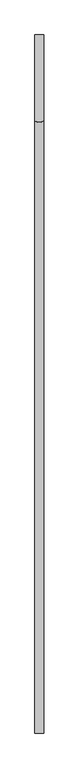
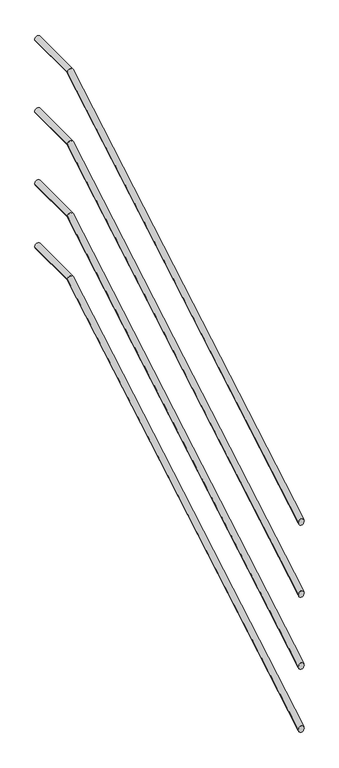
"""IFC4 building model written with IfcOpenShell, lengths in millimetres: railing geometry."""

import ifcopenshell
import ifcopenshell.guid

model = None  # the IFC model being written
_history = None  # IfcOwnerHistory: only IFC2X3 demands one
_inside = {}  # id of a spatial element -> (the spatial element, [elements in it])
_under = {}  # id of a project, library or spatial element -> (it, [spatial elements below it])
_declared = {}  # id of a project -> (the project, [libraries it declares])
_typed = {}  # id of a type object -> (the type object, [elements of that type])
_made_of = {}  # id of a material, layer set ... -> (it, [elements and type objects made of it])


def new_model(schema):
    """Start an empty IFC model of exactly this schema.

    Asked for "IFC4X3", IfcOpenShell would pick the latest addendum, in which some entities
    have other attributes; the version numbers below select the first issue.
    IFC2X3 requires an IfcOwnerHistory on every rooted entity: one is made here for all.
    """
    global model, _history
    if schema == "IFC4X3":
        model = ifcopenshell.file(schema_version=(4, 3, 0, 0))
    else:
        model = ifcopenshell.file(schema=schema)
    _inside.clear()
    _under.clear()
    _declared.clear()
    _typed.clear()
    _made_of.clear()
    _history = None
    if model.schema == "IFC2X3":
        org = make("IfcOrganization", Name="unknown")
        user = make(
            "IfcPersonAndOrganization",
            ThePerson=make("IfcPerson", FamilyName="unknown"),
            TheOrganization=org,
        )
        app = make(
            "IfcApplication",
            ApplicationDeveloper=org,
            Version="unknown",
            ApplicationFullName="unknown",
            ApplicationIdentifier="unknown",
        )
        _history = make(
            "IfcOwnerHistory",
            OwningUser=user,
            OwningApplication=app,
            ChangeAction="ADDED",
            CreationDate=0,
        )
    return model


def make(cls, **values):
    """One entity of the class cls with the attributes given. An attribute that is None is left unset."""
    return model.create_entity(
        cls, **{name: value for name, value in values.items() if value is not None}
    )


def rooted(cls, **values):
    """An entity with a GlobalId (a new one), such as an element, a storey or a relation."""
    return make(cls, GlobalId=ifcopenshell.guid.new(), OwnerHistory=_history, **values)


def si_unit(unit_type, name, prefix=None):
    """IfcSIUnit, for example si_unit("LENGTHUNIT", "METRE", prefix="MILLI")."""
    return make("IfcSIUnit", UnitType=unit_type, Prefix=prefix, Name=name)


def assignment(units):
    """IfcUnitAssignment: the units of a project."""
    return None if units is None else make("IfcUnitAssignment", Units=units)


def point(xyz):
    """IfcCartesianPoint."""
    return None if xyz is None else make("IfcCartesianPoint", Coordinates=xyz)


def direction(xyz):
    """IfcDirection."""
    return None if xyz is None else make("IfcDirection", DirectionRatios=xyz)


def frame(location, z_axis=None, x_axis=None):
    """IfcAxis2Placement3D, a coordinate frame: its origin and axes. An axis left out is left unset."""
    return make(
        "IfcAxis2Placement3D",
        Location=point(location),
        Axis=direction(z_axis),
        RefDirection=direction(x_axis),
    )


def origin():
    """The frame at (0, 0, 0) with its axes left unset."""
    return frame((0.0, 0.0, 0.0))


def place(relative_to, where):
    """IfcLocalPlacement: puts the frame where relative to a parent placement (None: the world)."""
    return make(
        "IfcLocalPlacement", PlacementRelTo=relative_to, RelativePlacement=where
    )


def context(
    kind, dimensions, precision=None, world=None, true_north=None, identifier=None
):
    """IfcGeometricRepresentationContext, for example the 3D "Model" context."""
    return make(
        "IfcGeometricRepresentationContext",
        ContextIdentifier=identifier,
        ContextType=kind,
        CoordinateSpaceDimension=dimensions,
        Precision=precision,
        WorldCoordinateSystem=world,
        TrueNorth=true_north,
    )


def project(units=None, contexts=None):
    """IfcProject with its units and contexts."""
    return rooted(
        "IfcProject",
        Name="project",
        RepresentationContexts=contexts,
        UnitsInContext=assignment(units),
    )


def spatial(cls, under=None, at=None, **own):
    """A site, building, storey or space (cls), placed at a placement, below another one or the project."""
    s = rooted(cls, ObjectPlacement=at, **own)
    if under is not None:
        _under.setdefault(under.id(), (under, []))[1].append(s)
    return s


def circle_curve(where, radius):
    """IfcCircle in the frame where."""
    return make("IfcCircle", Position=where, Radius=radius)


def ellipse_curve(where, semi_axis1, semi_axis2):
    """IfcEllipse in the frame where."""
    return make(
        "IfcEllipse", Position=where, SemiAxis1=semi_axis1, SemiAxis2=semi_axis2
    )


def shape(context_of_items, identifier, shape_type, items):
    """IfcShapeRepresentation: the items that make up one representation, for example the "Body"."""
    return make(
        "IfcShapeRepresentation",
        ContextOfItems=context_of_items,
        RepresentationIdentifier=identifier,
        RepresentationType=shape_type,
        Items=items,
    )


def source(mapping_origin, context_of_items, identifier, shape_type, items):
    """IfcRepresentationMap: a shape defined once, which mapped items show again and again."""
    return make(
        "IfcRepresentationMap",
        MappingOrigin=mapping_origin,
        MappedRepresentation=shape(context_of_items, identifier, shape_type, items),
    )


def transform(
    local_origin,
    x_axis=None,
    y_axis=None,
    z_axis=None,
    scale=None,
    scale2=None,
    scale3=None,
    uniform=True,
):
    """IfcCartesianTransformationOperator3D, or its non-uniform kind. x_axis, y_axis, z_axis: its Axis1, 2, 3."""
    if uniform:
        return make(
            "IfcCartesianTransformationOperator3D",
            Axis1=direction(x_axis),
            Axis2=direction(y_axis),
            LocalOrigin=point(local_origin),
            Scale=scale,
            Axis3=direction(z_axis),
        )
    return make(
        "IfcCartesianTransformationOperator3DnonUniform",
        Axis1=direction(x_axis),
        Axis2=direction(y_axis),
        LocalOrigin=point(local_origin),
        Scale=scale,
        Axis3=direction(z_axis),
        Scale2=scale2,
        Scale3=scale3,
    )


def mapped(mapping_source, mapping_target):
    """IfcMappedItem: shows the shape of a source again, moved by a transform."""
    return make(
        "IfcMappedItem", MappingSource=mapping_source, MappingTarget=mapping_target
    )


def made_of(thing, what):
    """Note that an element or type object is made of a material, layer set ...; save() writes the relation."""
    if what is not None:
        _made_of.setdefault(what.id(), (what, []))[1].append(thing)
    return thing


def element(
    cls,
    number,
    at=None,
    inside=None,
    cuts=None,
    type_object=None,
    material=None,
    context=None,
    identifier="Body",
    shape_type=None,
    held_by="IfcProductDefinitionShape",
    body=None,
    shapes=None,
    **own,
):
    """One element of the class cls, such as IfcWall. Its Tag is "e" and its number.

    at: its placement. inside: the storey or other place that contains it. cuts: it is an
    opening in that element (IfcRelVoidsElement). A single representation is given by context,
    identifier, shape_type and body (its items); several are given by shapes. held_by: the class
    of the entity that holds the representations. save() writes the other relations.
    """
    e = rooted(cls, Tag="e%d" % number, ObjectPlacement=at, **own)
    if body is not None:
        shapes = [shape(context, identifier, shape_type, body)]
    if shapes is not None:
        e.Representation = make(held_by, Representations=shapes)
    if inside is not None:
        _inside.setdefault(inside.id(), (inside, []))[1].append(e)
    if cuts is not None:
        rooted(
            "IfcRelVoidsElement", RelatingBuildingElement=cuts, RelatedOpeningElement=e
        )
    if type_object is not None:
        _typed.setdefault(type_object.id(), (type_object, []))[1].append(e)
    return made_of(e, material)


def aggregate(whole, parts):
    """IfcRelAggregates: a whole, such as a stair, and the parts it consists of."""
    return rooted("IfcRelAggregates", RelatingObject=whole, RelatedObjects=parts)


def save(model, path):
    """Write the relations noted so far, then the file.

    IfcRelAggregates (storeys below a building ...), IfcRelContainedInSpatialStructure (elements
    in a storey), IfcRelDefinesByType, IfcRelAssociatesMaterial and IfcRelDeclares: one each for
    every whole, place, type object, material and project.
    """
    for whole, parts in _under.values():
        aggregate(whole, parts)
    for where, things in _inside.values():
        rooted(
            "IfcRelContainedInSpatialStructure",
            RelatedElements=things,
            RelatingStructure=where,
        )
    for kind, things in _typed.values():
        rooted("IfcRelDefinesByType", RelatedObjects=things, RelatingType=kind)
    for what, things in _made_of.values():
        rooted("IfcRelAssociatesMaterial", RelatedObjects=things, RelatingMaterial=what)
    for by, libraries in _declared.values():
        rooted("IfcRelDeclares", RelatingContext=by, RelatedDefinitions=libraries)
    model.write(path)


def plane_surface(at):
    """IfcPlane: the flat surface through the origin of the frame at, square to its z axis."""
    return make("IfcPlane", Position=at)


def cylinder_surface(at, radius):
    """IfcCylindricalSurface: all points at the distance radius from the z axis of the frame at."""
    return make("IfcCylindricalSurface", Position=at, Radius=radius)


def advanced_brep(points, edges, surfaces, faces):
    """IfcAdvancedBrep: a solid bounded by faces that lie on surfaces and meet in shared edges.

    An edge is (start, end): straight between two places in points (the first is 0);
    or (start, end, curve); or (start, end, curve, False) where it runs against its curve.
    A face is (place in surfaces, loops), or (place, loops, False) where it looks against
    its surface's normal. A loop lists edges by number (the first is 1), with a minus sign
    where the edge is run from its end to its start. The first loop is the outer one.
    """
    corners = [point(p) for p in points]
    vertices = [make("IfcVertexPoint", VertexGeometry=c) for c in corners]
    made = []
    for start, end, *more in edges:
        made.append(
            make(
                "IfcEdgeCurve",
                EdgeStart=vertices[start],
                EdgeEnd=vertices[end],
                EdgeGeometry=more[0] if more else make("IfcPolyline", Points=[corners[start], corners[end]]),
                SameSense=more[1] if len(more) > 1 else True,
            )
        )
    hull = []
    for where, loops, *sense in faces:
        bounds = []
        for j, loop in enumerate(loops):
            ring = [make("IfcOrientedEdge", EdgeElement=made[abs(k) - 1], Orientation=k > 0) for k in loop]
            bounds.append(
                make(
                    "IfcFaceOuterBound" if j == 0 else "IfcFaceBound",
                    Bound=make("IfcEdgeLoop", EdgeList=ring),
                    Orientation=True,
                )
            )
        hull.append(make("IfcAdvancedFace", Bounds=bounds, FaceSurface=surfaces[where], SameSense=sense[0] if sense else True))
    return make("IfcAdvancedBrep", Outer=make("IfcClosedShell", CfsFaces=hull))


def railing_ea222afd(model_context):
    return source(origin(), model_context, "Body", "AdvancedBrep", [
        advanced_brep(
        [(-3259.6, 13399.5208589, 7257.5963084), (-3289.6, 13399.5208589, 7257.5963084), (-3259.6, 15503.576096, 8484.9618634), (-3289.6, 15503.576096, 8484.9618634), (-3259.6, 15799.5208589, 8484.9618634), (-3289.6, 15799.5208589, 8484.9618634)],
        [
            (0, 1, ellipse_curve(frame((-3274.6, 13399.5208589, 7257.5963084), z_axis=(0.0, -1.0, 0.0), x_axis=(0.0, 0.0, -1.0)), 17.365555, 15.0)),
            (1, 0, ellipse_curve(frame((-3274.6, 13399.5208589, 7257.5963084), z_axis=(0.0, -1.0, 0.0), x_axis=(0.0, 0.0, -1.0)), 17.365555, 15.0)),
            (0, 2),
            (2, 3, ellipse_curve(frame((-3274.6, 15503.576096, 8484.9618634), z_axis=(0.0, -0.9653442134540492, -0.26097997921446614), x_axis=(0.0, 0.26097997921446614, -0.9653442134540491)), 15.5384989, 15.0)),
            (3, 1),
            (3, 2, ellipse_curve(frame((-3274.6, 15503.576096, 8484.9618634), z_axis=(0.0, -0.9653442134540492, -0.26097997921446614), x_axis=(0.0, 0.26097997921446614, -0.9653442134540491)), 15.5384989, 15.0)),
            (4, 5, circle_curve(frame((-3274.6, 15799.5208589, 8484.9618634), z_axis=(0.0, 1.0, 0.0), x_axis=(-1.0, 0.0, 0.0)), 15.0)),
            (5, 4, circle_curve(frame((-3274.6, 15799.5208589, 8484.9618634), z_axis=(0.0, 1.0, 0.0), x_axis=(-1.0, 0.0, 0.0)), 15.0)),
            (2, 4),
            (5, 3),
        ],
        [
            plane_surface(frame((-3274.6, 13399.5208589, 7274.9618634), z_axis=(0.0, -1.0, 0.0), x_axis=(0.0, 0.0, 1.0))),
            cylinder_surface(frame((-3274.6, 13407.0789243, 7262.0051799), z_axis=(0.0, -0.8637789008984336, -0.5038710255240859), x_axis=(-1.0, 0.0, 0.0)), 15.0),
            plane_surface(frame((-3274.6, 15799.5208589, 8499.9618634), z_axis=(0.0, 1.0, 0.0), x_axis=(0.0, 0.0, 1.0))),
            cylinder_surface(frame((-3274.6, 15499.5208589, 8484.9618634), z_axis=(0.0, -1.0, 0.0), x_axis=(-1.0, 0.0, 0.0)), 15.0),
        ],
        [
            (0, [[1, 2]]),
            (1, [[-1, 3, 4, 5]]),
            (1, [[-2, -5, 6, -3]]),
            (2, [[7, 8]]),
            (3, [[-4, 9, -8, 10]]),
            (3, [[-6, -10, -7, -9]]),
        ],
    ),
        advanced_brep(
        [(-3259.6, 13399.5208589, 6457.5963084), (-3289.6, 13399.5208589, 6457.5963084), (-3259.6, 15503.576096, 7684.9618634), (-3289.6, 15503.576096, 7684.9618634), (-3259.6, 15799.5208589, 7684.9618634), (-3289.6, 15799.5208589, 7684.9618634)],
        [
            (0, 1, ellipse_curve(frame((-3274.6, 13399.5208589, 6457.5963084), z_axis=(0.0, -1.0, 0.0), x_axis=(0.0, 0.0, -1.0)), 17.365555, 15.0)),
            (1, 0, ellipse_curve(frame((-3274.6, 13399.5208589, 6457.5963084), z_axis=(0.0, -1.0, 0.0), x_axis=(0.0, 0.0, -1.0)), 17.365555, 15.0)),
            (0, 2),
            (2, 3, ellipse_curve(frame((-3274.6, 15503.576096, 7684.9618634), z_axis=(0.0, -0.9653442134540492, -0.26097997921446614), x_axis=(0.0, 0.26097997921446614, -0.9653442134540491)), 15.5384989, 15.0)),
            (3, 1),
            (3, 2, ellipse_curve(frame((-3274.6, 15503.576096, 7684.9618634), z_axis=(0.0, -0.9653442134540492, -0.26097997921446614), x_axis=(0.0, 0.26097997921446614, -0.9653442134540491)), 15.5384989, 15.0)),
            (4, 5, circle_curve(frame((-3274.6, 15799.5208589, 7684.9618634), z_axis=(0.0, 1.0, 0.0), x_axis=(-1.0, 0.0, 0.0)), 15.0)),
            (5, 4, circle_curve(frame((-3274.6, 15799.5208589, 7684.9618634), z_axis=(0.0, 1.0, 0.0), x_axis=(-1.0, 0.0, 0.0)), 15.0)),
            (2, 4),
            (5, 3),
        ],
        [
            plane_surface(frame((-3274.6, 13399.5208589, 6474.9618634), z_axis=(0.0, -1.0, 0.0), x_axis=(0.0, 0.0, 1.0))),
            cylinder_surface(frame((-3274.6, 13407.0789243, 6462.0051799), z_axis=(0.0, -0.8637789008984336, -0.5038710255240859), x_axis=(-1.0, 0.0, 0.0)), 15.0),
            plane_surface(frame((-3274.6, 15799.5208589, 7699.9618634), z_axis=(0.0, 1.0, 0.0), x_axis=(0.0, 0.0, 1.0))),
            cylinder_surface(frame((-3274.6, 15499.5208589, 7684.9618634), z_axis=(0.0, -1.0, 0.0), x_axis=(-1.0, 0.0, 0.0)), 15.0),
        ],
        [
            (0, [[1, 2]]),
            (1, [[-1, 3, 4, 5]]),
            (1, [[-2, -5, 6, -3]]),
            (2, [[7, 8]]),
            (3, [[-4, 9, -8, 10]]),
            (3, [[-6, -10, -7, -9]]),
        ],
    ),
        advanced_brep(
        [(-3259.6, 13399.5208589, 6857.5963084), (-3289.6, 13399.5208589, 6857.5963084), (-3259.6, 15503.576096, 8084.9618634), (-3289.6, 15503.576096, 8084.9618634), (-3259.6, 15799.5208589, 8084.9618634), (-3289.6, 15799.5208589, 8084.9618634)],
        [
            (0, 1, ellipse_curve(frame((-3274.6, 13399.5208589, 6857.5963084), z_axis=(0.0, -1.0, 0.0), x_axis=(0.0, 0.0, -1.0)), 17.365555, 15.0)),
            (1, 0, ellipse_curve(frame((-3274.6, 13399.5208589, 6857.5963084), z_axis=(0.0, -1.0, 0.0), x_axis=(0.0, 0.0, -1.0)), 17.365555, 15.0)),
            (0, 2),
            (2, 3, ellipse_curve(frame((-3274.6, 15503.576096, 8084.9618634), z_axis=(0.0, -0.9653442134540492, -0.26097997921446614), x_axis=(0.0, 0.26097997921446614, -0.9653442134540491)), 15.5384989, 15.0)),
            (3, 1),
            (3, 2, ellipse_curve(frame((-3274.6, 15503.576096, 8084.9618634), z_axis=(0.0, -0.9653442134540492, -0.26097997921446614), x_axis=(0.0, 0.26097997921446614, -0.9653442134540491)), 15.5384989, 15.0)),
            (4, 5, circle_curve(frame((-3274.6, 15799.5208589, 8084.9618634), z_axis=(0.0, 1.0, 0.0), x_axis=(-1.0, 0.0, 0.0)), 15.0)),
            (5, 4, circle_curve(frame((-3274.6, 15799.5208589, 8084.9618634), z_axis=(0.0, 1.0, 0.0), x_axis=(-1.0, 0.0, 0.0)), 15.0)),
            (2, 4),
            (5, 3),
        ],
        [
            plane_surface(frame((-3274.6, 13399.5208589, 6874.9618634), z_axis=(0.0, -1.0, 0.0), x_axis=(0.0, 0.0, 1.0))),
            cylinder_surface(frame((-3274.6, 13407.0789243, 6862.0051799), z_axis=(0.0, -0.8637789008984336, -0.5038710255240859), x_axis=(-1.0, 0.0, 0.0)), 15.0),
            plane_surface(frame((-3274.6, 15799.5208589, 8099.9618634), z_axis=(0.0, 1.0, 0.0), x_axis=(0.0, 0.0, 1.0))),
            cylinder_surface(frame((-3274.6, 15499.5208589, 8084.9618634), z_axis=(0.0, -1.0, 0.0), x_axis=(-1.0, 0.0, 0.0)), 15.0),
        ],
        [
            (0, [[1, 2]]),
            (1, [[-1, 3, 4, 5]]),
            (1, [[-2, -5, 6, -3]]),
            (2, [[7, 8]]),
            (3, [[-4, 9, -8, 10]]),
            (3, [[-6, -10, -7, -9]]),
        ],
    ),
        advanced_brep(
        [(-3259.6, 13399.5208589, 6107.5963084), (-3289.6, 13399.5208589, 6107.5963084), (-3259.6, 15503.576096, 7334.9618634), (-3289.6, 15503.576096, 7334.9618634), (-3259.6, 15799.5208589, 7334.9618634), (-3289.6, 15799.5208589, 7334.9618634)],
        [
            (0, 1, ellipse_curve(frame((-3274.6, 13399.5208589, 6107.5963084), z_axis=(0.0, -1.0, 0.0), x_axis=(0.0, 0.0, -1.0)), 17.365555, 15.0)),
            (1, 0, ellipse_curve(frame((-3274.6, 13399.5208589, 6107.5963084), z_axis=(0.0, -1.0, 0.0), x_axis=(0.0, 0.0, -1.0)), 17.365555, 15.0)),
            (0, 2),
            (2, 3, ellipse_curve(frame((-3274.6, 15503.576096, 7334.9618634), z_axis=(0.0, -0.9653442134540492, -0.26097997921446614), x_axis=(0.0, 0.26097997921446614, -0.9653442134540491)), 15.5384989, 15.0)),
            (3, 1),
            (3, 2, ellipse_curve(frame((-3274.6, 15503.576096, 7334.9618634), z_axis=(0.0, -0.9653442134540492, -0.26097997921446614), x_axis=(0.0, 0.26097997921446614, -0.9653442134540491)), 15.5384989, 15.0)),
            (4, 5, circle_curve(frame((-3274.6, 15799.5208589, 7334.9618634), z_axis=(0.0, 1.0, 0.0), x_axis=(-1.0, 0.0, 0.0)), 15.0)),
            (5, 4, circle_curve(frame((-3274.6, 15799.5208589, 7334.9618634), z_axis=(0.0, 1.0, 0.0), x_axis=(-1.0, 0.0, 0.0)), 15.0)),
            (2, 4),
            (5, 3),
        ],
        [
            plane_surface(frame((-3274.6, 13399.5208589, 6124.9618634), z_axis=(0.0, -1.0, 0.0), x_axis=(0.0, 0.0, 1.0))),
            cylinder_surface(frame((-3274.6, 13407.0789243, 6112.0051799), z_axis=(0.0, -0.8637789008984336, -0.5038710255240859), x_axis=(-1.0, 0.0, 0.0)), 15.0),
            plane_surface(frame((-3274.6, 15799.5208589, 7349.9618634), z_axis=(0.0, 1.0, 0.0), x_axis=(0.0, 0.0, 1.0))),
            cylinder_surface(frame((-3274.6, 15499.5208589, 7334.9618634), z_axis=(0.0, -1.0, 0.0), x_axis=(-1.0, 0.0, 0.0)), 15.0),
        ],
        [
            (0, [[1, 2]]),
            (1, [[-1, 3, 4, 5]]),
            (1, [[-2, -5, 6, -3]]),
            (2, [[7, 8]]),
            (3, [[-4, 9, -8, 10]]),
            (3, [[-6, -10, -7, -9]]),
        ],
    ),
    ])


if __name__ == "__main__":
    model = new_model("IFC4")
    model_context = context("Model", 3, world=origin())
    ifc_project = project(units=[si_unit("LENGTHUNIT", "METRE", prefix="MILLI")], contexts=[model_context])
    site = spatial("IfcSite", under=ifc_project)
    building = spatial("IfcBuilding", under=site)
    placement = place(None, origin())
    railing_shape = railing_ea222afd(model_context)
    element("IfcRailing", 1, at=placement, inside=building, context=model_context, shape_type="MappedRepresentation", body=[
        mapped(railing_shape, transform((0.0, 0.0, 0.0), x_axis=(1.0, 0.0, 0.0), y_axis=(0.0, 1.0, 0.0), z_axis=(0.0, 0.0, 1.0))),
    ])
    save(model, "model.ifc")
